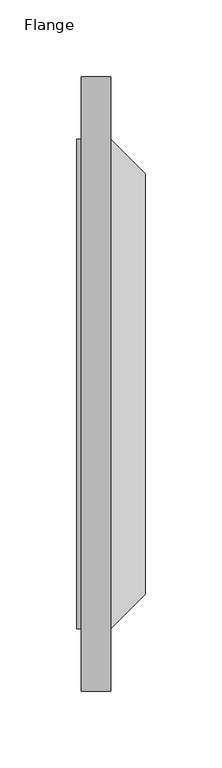
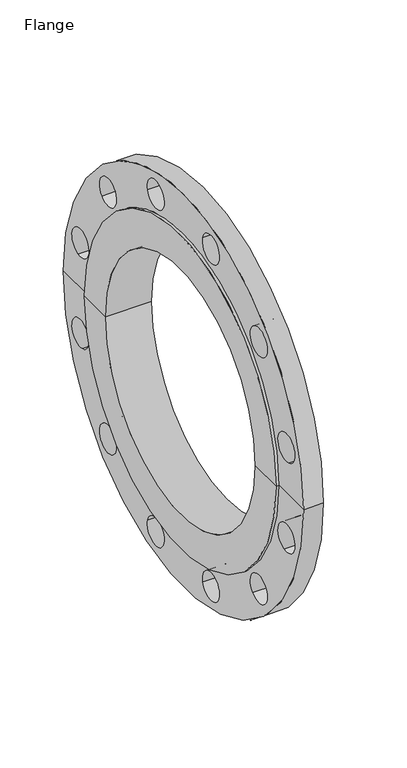
"""IFC4 building model written with IfcOpenShell, lengths in millimetres: proxy geometry, Flange : CASTED FLANGE PN16."""

from ifc_helpers import new_model, si_unit, frame, origin, place, context, project, spatial, polyline, circle_curve, source, transform, mapped, element, save
from ifc_brep_helpers import plane_surface, cylinder_surface, revolved_surface, advanced_brep


def flange_cf0ee467(model_context):
    return source(origin(), model_context, "Body", "AdvancedBrep", [
        advanced_brep(
        [(0.0, -125.0, 0.0), (0.0, 125.0, 0.0), (0.0, 159.5, 0.0), (0.0, -159.5, 0.0), (44.5, -125.0, 0.0), (44.5, 125.0, 0.0), (44.5, -137.0, 0.0), (44.5, 137.0, 0.0), (22.0, -159.5, 0.0), (22.0, 159.5, 0.0), (22.0, -200.0, 0.0), (22.0, 200.0, 0.0), (22.0, 59.4633421, -167.8283675), (22.0, 32.4174189, -175.0753008), (22.0, -32.4174189, -175.0753008), (22.0, -59.4633421, -167.8283675), (22.0, 135.4109486, -115.6119587), (22.0, 115.6119587, -135.4109486), (22.0, 175.0753008, -32.4174189), (22.0, 167.8283675, -59.4633421), (22.0, -167.8283675, -59.4633421), (22.0, -175.0753008, -32.4174189), (22.0, -115.6119587, -135.4109486), (22.0, -135.4109486, -115.6119587), (22.0, 32.4174189, 175.0753008), (22.0, 59.4633421, 167.8283675), (22.0, -59.4633421, 167.8283675), (22.0, -32.4174189, 175.0753008), (22.0, 167.8283675, 59.4633421), (22.0, 175.0753008, 32.4174189), (22.0, 115.6119587, 135.4109486), (22.0, 135.4109486, 115.6119587), (22.0, -135.4109486, 115.6119587), (22.0, -115.6119587, 135.4109486), (22.0, -175.0753008, 32.4174189), (22.0, -167.8283675, 59.4633421), (3.0, -200.0, 0.0), (3.0, 200.0, 0.0), (3.0, -159.5, 0.0), (3.0, 159.5, 0.0), (3.0, 32.4174189, -175.0753008), (3.0, 59.4633421, -167.8283675), (3.0, -59.4633421, -167.8283675), (3.0, -32.4174189, -175.0753008), (3.0, 115.6119587, -135.4109486), (3.0, 135.4109486, -115.6119587), (3.0, 167.8283675, -59.4633421), (3.0, 175.0753008, -32.4174189), (3.0, -175.0753008, -32.4174189), (3.0, -167.8283675, -59.4633421), (3.0, -135.4109486, -115.6119587), (3.0, -115.6119587, -135.4109486), (3.0, 59.4633421, 167.8283675), (3.0, 32.4174189, 175.0753008), (3.0, -32.4174189, 175.0753008), (3.0, -59.4633421, 167.8283675), (3.0, 175.0753008, 32.4174189), (3.0, 167.8283675, 59.4633421), (3.0, 135.4109486, 115.6119587), (3.0, 115.6119587, 135.4109486), (3.0, -115.6119587, 135.4109486), (3.0, -135.4109486, 115.6119587), (3.0, -167.8283675, 59.4633421), (3.0, -175.0753008, 32.4174189)],
        [
            (0, 1, circle_curve(frame((0.0, 0.0, 0.0), z_axis=(1.0, 0.0, 0.0), x_axis=(0.0, -1.0, 0.0)), 125.0)),
            (1, 2),
            (2, 3, circle_curve(frame((0.0, 0.0, 0.0), z_axis=(-1.0, 0.0, 0.0), x_axis=(0.0, -1.0, 0.0)), 159.5)),
            (3, 0),
            (3, 2, circle_curve(frame((0.0, 0.0, 0.0), z_axis=(-1.0, 0.0, 0.0), x_axis=(0.0, -1.0, 0.0)), 159.5)),
            (1, 0, circle_curve(frame((0.0, 0.0, 0.0), z_axis=(1.0, 0.0, 0.0), x_axis=(0.0, -1.0, 0.0)), 125.0)),
            (4, 5, circle_curve(frame((44.5, 0.0, 0.0), z_axis=(1.0, 0.0, 0.0), x_axis=(0.0, -1.0, 0.0)), 125.0)),
            (5, 1),
            (0, 4),
            (5, 4, circle_curve(frame((44.5, 0.0, 0.0), z_axis=(1.0, 0.0, 0.0), x_axis=(0.0, -1.0, 0.0)), 125.0)),
            (6, 7, circle_curve(frame((44.5, 0.0, 0.0), z_axis=(1.0, 0.0, 0.0), x_axis=(0.0, -1.0, 0.0)), 137.0)),
            (7, 5),
            (4, 6),
            (7, 6, circle_curve(frame((44.5, 0.0, 0.0), z_axis=(1.0, 0.0, 0.0), x_axis=(0.0, -1.0, 0.0)), 137.0)),
            (8, 9, circle_curve(frame((22.0, 0.0, 0.0), z_axis=(1.0, 0.0, 0.0), x_axis=(0.0, -1.0, 0.0)), 159.5)),
            (9, 7),
            (6, 8),
            (9, 8, circle_curve(frame((22.0, 0.0, 0.0), z_axis=(1.0, 0.0, 0.0), x_axis=(0.0, -1.0, 0.0)), 159.5)),
            (10, 11, circle_curve(frame((22.0, 0.0, 0.0), z_axis=(1.0, 0.0, 0.0), x_axis=(0.0, -1.0, 0.0)), 200.0)),
            (11, 9),
            (8, 10),
            (12, 13, circle_curve(frame((22.0, 45.9403805, -171.4518342), z_axis=(-1.0, 0.0, 0.0), x_axis=(0.0, -0.9659258262890734, -0.258819045102502)), 14.0)),
            (13, 12, circle_curve(frame((22.0, 45.9403805, -171.4518342), z_axis=(-1.0, 0.0, 0.0), x_axis=(0.0, -0.9659258262890734, -0.258819045102502)), 14.0)),
            (14, 15, circle_curve(frame((22.0, -45.9403805, -171.4518342), z_axis=(-1.0, 0.0, 0.0), x_axis=(0.0, -0.9659258262890654, 0.25881904510253184)), 14.0)),
            (15, 14, circle_curve(frame((22.0, -45.9403805, -171.4518342), z_axis=(-1.0, 0.0, 0.0), x_axis=(0.0, -0.9659258262890654, 0.25881904510253184)), 14.0)),
            (16, 17, circle_curve(frame((22.0, 125.5114537, -125.5114537), z_axis=(-1.0, 0.0, 0.0), x_axis=(0.0, -0.7071067811865748, -0.7071067811865202)), 14.0)),
            (17, 16, circle_curve(frame((22.0, 125.5114537, -125.5114537), z_axis=(-1.0, 0.0, 0.0), x_axis=(0.0, -0.7071067811865748, -0.7071067811865202)), 14.0)),
            (18, 19, circle_curve(frame((22.0, 171.4518342, -45.9403805), z_axis=(-1.0, 0.0, 0.0), x_axis=(0.0, -0.25881904510254733, -0.9659258262890613)), 14.0)),
            (19, 18, circle_curve(frame((22.0, 171.4518342, -45.9403805), z_axis=(-1.0, 0.0, 0.0), x_axis=(0.0, -0.25881904510254733, -0.9659258262890613)), 14.0)),
            (20, 21, circle_curve(frame((22.0, -171.4518342, -45.9403805), z_axis=(-1.0, 0.0, 0.0), x_axis=(0.0, -0.2588190451024855, 0.9659258262890777)), 14.0)),
            (21, 20, circle_curve(frame((22.0, -171.4518342, -45.9403805), z_axis=(-1.0, 0.0, 0.0), x_axis=(0.0, -0.2588190451024855, 0.9659258262890777)), 14.0)),
            (22, 23, circle_curve(frame((22.0, -125.5114537, -125.5114537), z_axis=(-1.0, 0.0, 0.0), x_axis=(0.0, -0.7071067811865215, 0.7071067811865739)), 14.0)),
            (23, 22, circle_curve(frame((22.0, -125.5114537, -125.5114537), z_axis=(-1.0, 0.0, 0.0), x_axis=(0.0, -0.7071067811865215, 0.7071067811865739)), 14.0)),
            (11, 10, circle_curve(frame((22.0, 0.0, 0.0), z_axis=(1.0, 0.0, 0.0), x_axis=(0.0, -1.0, 0.0)), 200.0)),
            (24, 25, circle_curve(frame((22.0, 45.9403805, 171.4518342), z_axis=(-1.0, 0.0, 0.0), x_axis=(0.0, 0.9659258262890627, -0.258819045102542)), 14.0)),
            (25, 24, circle_curve(frame((22.0, 45.9403805, 171.4518342), z_axis=(-1.0, 0.0, 0.0), x_axis=(0.0, 0.9659258262890627, -0.258819045102542)), 14.0)),
            (26, 27, circle_curve(frame((22.0, -45.9403805, 171.4518342), z_axis=(-1.0, 0.0, 0.0), x_axis=(0.0, 0.9659258262890742, 0.25881904510249887)), 14.0)),
            (27, 26, circle_curve(frame((22.0, -45.9403805, 171.4518342), z_axis=(-1.0, 0.0, 0.0), x_axis=(0.0, 0.9659258262890742, 0.25881904510249887)), 14.0)),
            (28, 29, circle_curve(frame((22.0, 171.4518342, 45.9403805), z_axis=(-1.0, 0.0, 0.0), x_axis=(0.0, 0.25881904510250014, -0.9659258262890739)), 14.0)),
            (29, 28, circle_curve(frame((22.0, 171.4518342, 45.9403805), z_axis=(-1.0, 0.0, 0.0), x_axis=(0.0, 0.25881904510250014, -0.9659258262890739)), 14.0)),
            (30, 31, circle_curve(frame((22.0, 125.5114537, 125.5114537), z_axis=(-1.0, 0.0, 0.0), x_axis=(0.0, 0.7071067811865321, -0.7071067811865631)), 14.0)),
            (31, 30, circle_curve(frame((22.0, 125.5114537, 125.5114537), z_axis=(-1.0, 0.0, 0.0), x_axis=(0.0, 0.7071067811865321, -0.7071067811865631)), 14.0)),
            (32, 33, circle_curve(frame((22.0, -125.5114537, 125.5114537), z_axis=(-1.0, 0.0, 0.0), x_axis=(0.0, 0.7071067811865728, 0.7071067811865224)), 14.0)),
            (33, 32, circle_curve(frame((22.0, -125.5114537, 125.5114537), z_axis=(-1.0, 0.0, 0.0), x_axis=(0.0, 0.7071067811865728, 0.7071067811865224)), 14.0)),
            (34, 35, circle_curve(frame((22.0, -171.4518342, 45.9403805), z_axis=(-1.0, 0.0, 0.0), x_axis=(0.0, 0.25881904510255627, 0.9659258262890589)), 14.0)),
            (35, 34, circle_curve(frame((22.0, -171.4518342, 45.9403805), z_axis=(-1.0, 0.0, 0.0), x_axis=(0.0, 0.25881904510255627, 0.9659258262890589)), 14.0)),
            (36, 37, circle_curve(frame((3.0, 0.0, 0.0), z_axis=(1.0, 0.0, 0.0), x_axis=(0.0, -1.0, 0.0)), 200.0)),
            (37, 11),
            (10, 36),
            (37, 36, circle_curve(frame((3.0, 0.0, 0.0), z_axis=(1.0, 0.0, 0.0), x_axis=(0.0, -1.0, 0.0)), 200.0)),
            (38, 39, circle_curve(frame((3.0, 0.0, 0.0), z_axis=(1.0, 0.0, 0.0), x_axis=(0.0, -1.0, 0.0)), 159.5)),
            (39, 37),
            (36, 38),
            (40, 41, circle_curve(frame((3.0, 45.9403805, -171.4518342), z_axis=(1.0, 0.0, 0.0), x_axis=(0.0, -0.9659258262890734, -0.258819045102502)), 14.0)),
            (41, 40, circle_curve(frame((3.0, 45.9403805, -171.4518342), z_axis=(1.0, 0.0, 0.0), x_axis=(0.0, -0.9659258262890734, -0.258819045102502)), 14.0)),
            (42, 43, circle_curve(frame((3.0, -45.9403805, -171.4518342), z_axis=(1.0, 0.0, 0.0), x_axis=(0.0, -0.9659258262890654, 0.25881904510253184)), 14.0)),
            (43, 42, circle_curve(frame((3.0, -45.9403805, -171.4518342), z_axis=(1.0, 0.0, 0.0), x_axis=(0.0, -0.9659258262890654, 0.25881904510253184)), 14.0)),
            (44, 45, circle_curve(frame((3.0, 125.5114537, -125.5114537), z_axis=(1.0, 0.0, 0.0), x_axis=(0.0, -0.7071067811865748, -0.7071067811865202)), 14.0)),
            (45, 44, circle_curve(frame((3.0, 125.5114537, -125.5114537), z_axis=(1.0, 0.0, 0.0), x_axis=(0.0, -0.7071067811865748, -0.7071067811865202)), 14.0)),
            (46, 47, circle_curve(frame((3.0, 171.4518342, -45.9403805), z_axis=(1.0, 0.0, 0.0), x_axis=(0.0, -0.25881904510254733, -0.9659258262890613)), 14.0)),
            (47, 46, circle_curve(frame((3.0, 171.4518342, -45.9403805), z_axis=(1.0, 0.0, 0.0), x_axis=(0.0, -0.25881904510254733, -0.9659258262890613)), 14.0)),
            (48, 49, circle_curve(frame((3.0, -171.4518342, -45.9403805), z_axis=(1.0, 0.0, 0.0), x_axis=(0.0, -0.2588190451024855, 0.9659258262890777)), 14.0)),
            (49, 48, circle_curve(frame((3.0, -171.4518342, -45.9403805), z_axis=(1.0, 0.0, 0.0), x_axis=(0.0, -0.2588190451024855, 0.9659258262890777)), 14.0)),
            (50, 51, circle_curve(frame((3.0, -125.5114537, -125.5114537), z_axis=(1.0, 0.0, 0.0), x_axis=(0.0, -0.7071067811865215, 0.7071067811865739)), 14.0)),
            (51, 50, circle_curve(frame((3.0, -125.5114537, -125.5114537), z_axis=(1.0, 0.0, 0.0), x_axis=(0.0, -0.7071067811865215, 0.7071067811865739)), 14.0)),
            (39, 38, circle_curve(frame((3.0, 0.0, 0.0), z_axis=(1.0, 0.0, 0.0), x_axis=(0.0, -1.0, 0.0)), 159.5)),
            (52, 53, circle_curve(frame((3.0, 45.9403805, 171.4518342), z_axis=(1.0, 0.0, 0.0), x_axis=(0.0, 0.9659258262890627, -0.258819045102542)), 14.0)),
            (53, 52, circle_curve(frame((3.0, 45.9403805, 171.4518342), z_axis=(1.0, 0.0, 0.0), x_axis=(0.0, 0.9659258262890627, -0.258819045102542)), 14.0)),
            (54, 55, circle_curve(frame((3.0, -45.9403805, 171.4518342), z_axis=(1.0, 0.0, 0.0), x_axis=(0.0, 0.9659258262890742, 0.25881904510249887)), 14.0)),
            (55, 54, circle_curve(frame((3.0, -45.9403805, 171.4518342), z_axis=(1.0, 0.0, 0.0), x_axis=(0.0, 0.9659258262890742, 0.25881904510249887)), 14.0)),
            (56, 57, circle_curve(frame((3.0, 171.4518342, 45.9403805), z_axis=(1.0, 0.0, 0.0), x_axis=(0.0, 0.25881904510250014, -0.9659258262890739)), 14.0)),
            (57, 56, circle_curve(frame((3.0, 171.4518342, 45.9403805), z_axis=(1.0, 0.0, 0.0), x_axis=(0.0, 0.25881904510250014, -0.9659258262890739)), 14.0)),
            (58, 59, circle_curve(frame((3.0, 125.5114537, 125.5114537), z_axis=(1.0, 0.0, 0.0), x_axis=(0.0, 0.7071067811865321, -0.7071067811865631)), 14.0)),
            (59, 58, circle_curve(frame((3.0, 125.5114537, 125.5114537), z_axis=(1.0, 0.0, 0.0), x_axis=(0.0, 0.7071067811865321, -0.7071067811865631)), 14.0)),
            (60, 61, circle_curve(frame((3.0, -125.5114537, 125.5114537), z_axis=(1.0, 0.0, 0.0), x_axis=(0.0, 0.7071067811865728, 0.7071067811865224)), 14.0)),
            (61, 60, circle_curve(frame((3.0, -125.5114537, 125.5114537), z_axis=(1.0, 0.0, 0.0), x_axis=(0.0, 0.7071067811865728, 0.7071067811865224)), 14.0)),
            (62, 63, circle_curve(frame((3.0, -171.4518342, 45.9403805), z_axis=(1.0, 0.0, 0.0), x_axis=(0.0, 0.25881904510255627, 0.9659258262890589)), 14.0)),
            (63, 62, circle_curve(frame((3.0, -171.4518342, 45.9403805), z_axis=(1.0, 0.0, 0.0), x_axis=(0.0, 0.25881904510255627, 0.9659258262890589)), 14.0)),
            (2, 39),
            (38, 3),
            (13, 40),
            (41, 12),
            (15, 42),
            (43, 14),
            (17, 44),
            (45, 16),
            (19, 46),
            (47, 18),
            (29, 56),
            (57, 28),
            (31, 58),
            (59, 30),
            (25, 52),
            (53, 24),
            (27, 54),
            (55, 26),
            (33, 60),
            (61, 32),
            (35, 62),
            (63, 34),
            (21, 48),
            (49, 20),
            (23, 50),
            (51, 22),
        ],
        [
            plane_surface(frame((0.0, 0.0, 0.0), z_axis=(-1.0, 0.0, 0.0), x_axis=(0.0, -1.0, 0.0))),
            revolved_surface(polyline([(0.0, -125.0, 0.0), (44.5, -125.0, 0.0)]), (-95.0, 0.0, 0.0), (-1.0, 0.0, 0.0)),
            plane_surface(frame((44.5, 0.0, 0.0), z_axis=(1.0, 0.0, 0.0), x_axis=(0.0, -1.0, 0.0))),
            revolved_surface(polyline([(44.5, -137.0, 0.0), (22.0, -159.5, 0.0)]), (-95.0, 0.0, 0.0), (-1.0, 0.0, 0.0)),
            plane_surface(frame((22.0, 0.0, 0.0), z_axis=(1.0, 0.0, 0.0), x_axis=(0.0, -1.0, 0.0))),
            cylinder_surface(frame((-95.0, 0.0, 0.0), z_axis=(-1.0, 0.0, 0.0), x_axis=(0.0, -1.0, 0.0)), 200.0),
            plane_surface(frame((3.0, 0.0, 0.0), z_axis=(-1.0, 0.0, 0.0), x_axis=(0.0, -1.0, 0.0))),
            cylinder_surface(frame((-95.0, 0.0, 0.0), z_axis=(-1.0, 0.0, 0.0), x_axis=(0.0, -1.0, 0.0)), 159.5),
            revolved_surface(polyline([(3.0, 32.41741893195297, -175.07530083143504), (22.0, 32.41741893195297, -175.07530083143504)]), (22.0, 45.9403805, -171.4518342), (-1.0, 0.0, 0.0)),
            revolved_surface(polyline([(3.0, -59.46334206804692, -167.82836756856457), (22.0, -59.46334206804692, -167.82836756856457)]), (22.0, -45.9403805, -171.4518342), (-1.0, 0.0, 0.0)),
            revolved_surface(polyline([(3.000000000000007, 115.61195876338796, -135.4109486366113), (22.0, 115.61195876338796, -135.4109486366113)]), (22.0, 125.5114537, -125.5114537), (-0.9999999999999998, 0.0, 0.0)),
            revolved_surface(polyline([(2.999999999999993, 167.82836756856435, -59.46334206804686), (22.0, 167.82836756856435, -59.46334206804686)]), (22.0, 171.4518342, -45.9403805), (-1.0000000000000002, 0.0, 0.0)),
            revolved_surface(polyline([(3.0, 175.07530083143502, 32.417418931952966), (22.0, 175.07530083143502, 32.417418931952966)]), (22.0, 171.4518342, 45.9403805), (-1.0, 0.0, 0.0)),
            revolved_surface(polyline([(3.0, 135.41094863661147, 115.61195876338812), (22.0, 135.41094863661147, 115.61195876338812)]), (22.0, 125.5114537, 125.5114537), (-1.0, 0.0, 0.0)),
            revolved_surface(polyline([(3.0, 59.463342068046884, 167.82836756856443), (22.0, 59.463342068046884, 167.82836756856443)]), (22.0, 45.9403805, 171.4518342), (-1.0, 0.0, 0.0)),
            revolved_surface(polyline([(3.0, -32.417418931952966, 175.075300831435), (22.0, -32.417418931952966, 175.075300831435)]), (22.0, -45.9403805, 171.4518342), (-1.0, 0.0, 0.0)),
            revolved_surface(polyline([(3.0, -115.61195876338799, 135.41094863661132), (22.0, -115.61195876338799, 135.41094863661132)]), (22.0, -125.5114537, 125.5114537), (-1.0, 0.0, 0.0)),
            revolved_surface(polyline([(3.0, -167.82836756856423, 59.46334206804683), (22.0, -167.82836756856423, 59.46334206804683)]), (22.0, -171.4518342, 45.9403805), (-1.0, 0.0, 0.0)),
            revolved_surface(polyline([(3.0, -175.07530083143482, -32.417418931952916), (22.0, -175.07530083143482, -32.417418931952916)]), (22.0, -171.4518342, -45.9403805), (-1.0, 0.0, 0.0)),
            revolved_surface(polyline([(2.999999999999993, -135.4109486366113, -115.61195876338797), (22.0, -135.4109486366113, -115.61195876338797)]), (22.0, -125.5114537, -125.5114537), (-1.0000000000000002, 0.0, 0.0)),
        ],
        [
            (0, [[1, 2, 3, 4]]),
            (0, [[5, -2, 6, -4]]),
            (1, [[7, 8, -1, 9]]),
            (1, [[-6, -8, 10, -9]]),
            (2, [[11, 12, -7, 13]]),
            (2, [[-10, -12, 14, -13]]),
            (3, [[15, 16, -11, 17]]),
            (3, [[-14, -16, 18, -17]]),
            (4, [[19, 20, -15, 21], [22, 23], [24, 25], [26, 27], [28, 29], [30, 31], [32, 33]]),
            (4, [[-18, -20, 34, -21], [35, 36], [37, 38], [39, 40], [41, 42], [43, 44], [45, 46]]),
            (5, [[47, 48, -19, 49]]),
            (5, [[-34, -48, 50, -49]]),
            (6, [[51, 52, -47, 53], [54, 55], [56, 57], [58, 59], [60, 61], [62, 63], [64, 65]]),
            (6, [[-50, -52, 66, -53], [67, 68], [69, 70], [71, 72], [73, 74], [75, 76], [77, 78]]),
            (7, [[-3, 79, -51, 80]]),
            (7, [[-66, -79, -5, -80]]),
            (8, [[-23, 81, -55, 82]]),
            (8, [[-54, -81, -22, -82]]),
            (9, [[-25, 83, -57, 84]]),
            (9, [[-56, -83, -24, -84]]),
            (10, [[-27, 85, -59, 86]]),
            (10, [[-58, -85, -26, -86]]),
            (11, [[-29, 87, -61, 88]]),
            (11, [[-60, -87, -28, -88]]),
            (12, [[-40, 89, -72, 90]]),
            (12, [[-71, -89, -39, -90]]),
            (13, [[-42, 91, -74, 92]]),
            (13, [[-73, -91, -41, -92]]),
            (14, [[-36, 93, -68, 94]]),
            (14, [[-67, -93, -35, -94]]),
            (15, [[-38, 95, -70, 96]]),
            (15, [[-69, -95, -37, -96]]),
            (16, [[-44, 97, -76, 98]]),
            (16, [[-75, -97, -43, -98]]),
            (17, [[-46, 99, -78, 100]]),
            (17, [[-77, -99, -45, -100]]),
            (18, [[-31, 101, -63, 102]]),
            (18, [[-62, -101, -30, -102]]),
            (19, [[-33, 103, -65, 104]]),
            (19, [[-64, -103, -32, -104]]),
        ],
    ),
    ])


if __name__ == "__main__":
    model = new_model("IFC4")
    model_context = context("Model", 3, world=origin())
    ifc_project = project(units=[si_unit("LENGTHUNIT", "METRE", prefix="MILLI")], contexts=[model_context])
    site = spatial("IfcSite", under=ifc_project)
    building = spatial("IfcBuilding", under=site)
    placement = place(None, origin())
    flange_shape = flange_cf0ee467(model_context)
    element("IfcBuildingElementProxy", 1, Name="Flange : CASTED FLANGE PN16", ObjectType="Flange : CASTED FLANGE PN16", at=placement, inside=building, context=model_context, shape_type="MappedRepresentation", body=[
        mapped(flange_shape, transform((0.0, 0.0, 0.0), x_axis=(1.0, 0.0, 0.0), y_axis=(0.0, 1.0, 0.0), z_axis=(0.0, 0.0, 1.0))),
    ])
    save(model, "model.ifc")

# Revit data of these elements
# Type "Flange : CASTED FLANGE PN16"
#   TABLE_DIMENSIONS = "DIMENSIONS FIXED FLANGE"
#   Short Description = ""
#   Description = "FIXED FLANGE"
#   K [instance default] = 110 mm
#   HOLE DIAMETER [instance default] = 19 mm
#   D4 [instance default] = 84 mm
#   DRILL DIAMETER [instance default] = 110 mm
#   DN [instance default] = 40 mm
#   D2 [instance default] = 70 mm
#   D [instance default] = 150 mm
#   f [instance default] = 3 mm
#   b [instance default] = 16 mm
#   ANGLE [instance default] = 45.00°
#   a [instance default] = 19 mm
#   PN = 16
#   BOLTS NUMBER [instance default] = 4
#   MATERIAL [instance default] = none
#   COATING [instance default] = none
#   Default Elevation = 0
# Element 1 (IfcBuildingElementProxy, "Flange : CASTED FLANGE PN16")
#   K = 355 mm
#   HOLE DIAMETER = 28 mm
#   D4 = 319 mm
#   DRILL DIAMETER = 355 mm
#   DN = 250 mm
#   D2 = 274 mm
#   D = 400 mm
#   b = 19 mm
#   a = 22 mm
#   BOLTS NUMBER = 12
#   COATING = Not informed
#   Materials on its faces: "Not informed"
# Materials
#   "Not informed": class "Paint/Coating", colour RGB 0 56 123, transparency 0, Description = "Not Informed", Cost = 0
